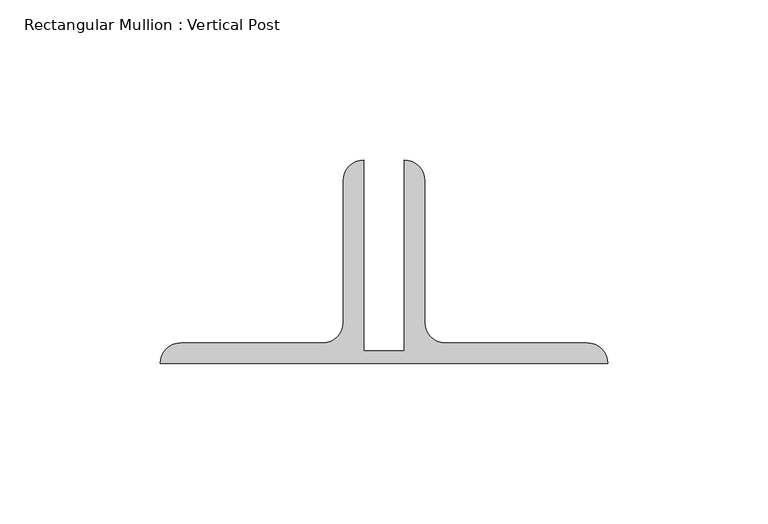
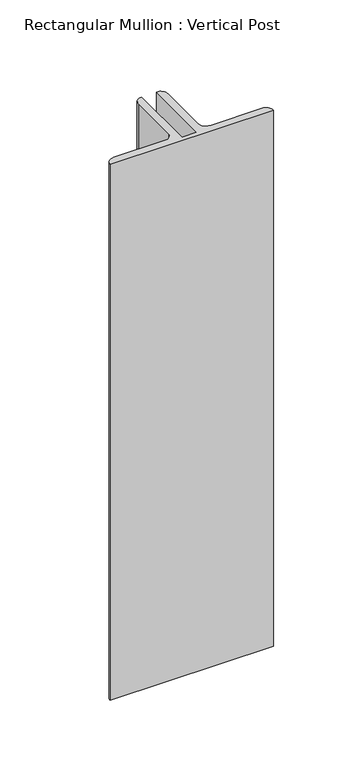
"""IFC4 building model written with IfcOpenShell, lengths in millimetres: member geometry, Rectangular Mullion : Vertical Post."""

from ifc_helpers import new_model, si_unit, point, frame, frame_2d, origin, place, context, project, spatial, polyline, circle_curve, trimmed, segment, composite_curve, outline, extrude, source, transform, mapped, element, save


def rectangular_mullion_vertical_post_e9d1dcc7(model_context):
    return source(origin(), model_context, "Body", "SweptSolid", [
        extrude(outline(composite_curve([segment(polyline([(-6.35, 22.9145205), (6.35, 22.9145205), (6.35, 82.55)]), True, "CONTINUOUS"), segment(trimmed(circle_curve(frame_2d((6.35, 76.2)), 6.35), [point((6.35, 82.55))], [point((12.7, 76.2))], False, "CARTESIAN"), True, "CONTINUOUS"), segment(polyline([(12.7, 76.2), (12.7, 31.75)]), True, "CONTINUOUS"), segment(trimmed(circle_curve(frame_2d((19.05, 31.75)), 6.35), [point((12.7, 31.75))], [point((19.05, 25.4))], True, "CARTESIAN"), True, "CONTINUOUS"), segment(polyline([(19.05, 25.4), (63.5, 25.4)]), True, "CONTINUOUS"), segment(trimmed(circle_curve(frame_2d((63.5, 19.05)), 6.35), [point((63.5, 25.4))], [point((69.85, 19.05))], False, "CARTESIAN"), True, "CONTINUOUS"), segment(polyline([(69.85, 19.05), (-69.85, 19.05)]), True, "CONTINUOUS"), segment(trimmed(circle_curve(frame_2d((-63.5, 19.05)), 6.35), [point((-69.85, 19.05))], [point((-63.5, 25.4))], False, "CARTESIAN"), True, "CONTINUOUS"), segment(polyline([(-63.5, 25.4), (-19.05, 25.4)]), True, "CONTINUOUS"), segment(trimmed(circle_curve(frame_2d((-19.05, 31.75)), 6.35), [point((-19.05, 25.4))], [point((-12.7, 31.75))], True, "CARTESIAN"), True, "CONTINUOUS"), segment(polyline([(-12.7, 31.75), (-12.7, 76.2)]), True, "CONTINUOUS"), segment(trimmed(circle_curve(frame_2d((-6.35, 76.2)), 6.35), [point((-12.7, 76.2))], [point((-6.35, 82.55))], False, "CARTESIAN"), True, "CONTINUOUS"), segment(polyline([(-6.35, 82.55), (-6.35, 22.9145205)]), True, "CONTINUOUS")], self_intersect=False)), frame((0.0, 0.0, -484.8663052), z_axis=(0.0, 0.0, 1.0), x_axis=(1.0, 0.0, 0.0)), (0.0, 0.0, 1.0), 484.8663052),
    ])


if __name__ == "__main__":
    model = new_model("IFC4")
    model_context = context("Model", 3, world=origin())
    ifc_project = project(units=[si_unit("LENGTHUNIT", "METRE", prefix="MILLI")], contexts=[model_context])
    site = spatial("IfcSite", under=ifc_project)
    building = spatial("IfcBuilding", under=site)
    placement = place(None, origin())
    rectangular_mullion_vertical_post_shape = rectangular_mullion_vertical_post_e9d1dcc7(model_context)
    element("IfcMember", 1, ObjectType="Rectangular Mullion : Vertical Post", at=placement, inside=building, context=model_context, shape_type="MappedRepresentation", body=[
        mapped(rectangular_mullion_vertical_post_shape, transform((0.0, 0.0, 0.0), x_axis=(1.0, 0.0, 0.0), y_axis=(0.0, 1.0, 0.0), z_axis=(0.0, 0.0, 1.0))),
    ])
    save(model, "model.ifc")

# Revit data of these elements
# Type "Rectangular Mullion : Vertical Post"
#   built-in parameter 1007351 = -0.0625 (stored number, unit not read)
#   built-in parameter 1007322 = 0.0126789 (stored number, unit not read)
#   built-in parameter 1007321 = 0.229167 (stored number, unit not read)
#   built-in parameter 1007320 = 0.229167 (stored number, unit not read)
# Element 1 (IfcMember, "Rectangular Mullion : Vertical Post")
#   Materials on its faces: "GATE POST: GALVANIZED ANGLES"
# Materials
#   "GATE POST: GALVANIZED ANGLES": class "Unassigned", colour RGB 120 120 120, transparency 0, Cost = 0
